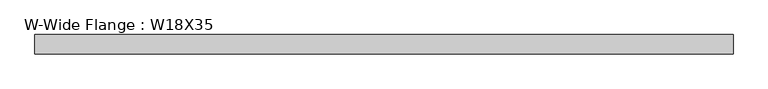
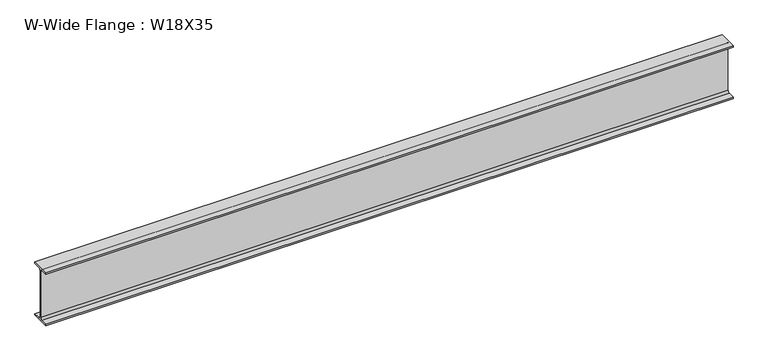
"""IFC4 building model written with IfcOpenShell, lengths in millimetres: beam geometry, W-Wide Flange : W18X35."""

from ifc_helpers import new_model, si_unit, point, frame, frame_2d, origin, place, context, project, spatial, polyline, circle_curve, trimmed, segment, composite_curve, outline, extrude, source, transform, mapped, element, save


def w_wide_flange_w18x35_70b9017d(model_context):
    return source(origin(), model_context, "Body", "SweptSolid", [
        extrude(outline(composite_curve([segment(polyline([(76.2, -213.995), (76.2, -224.79), (-76.2, -224.79), (-76.2, -213.995), (-21.59, -213.995)]), True, "CONTINUOUS"), segment(trimmed(circle_curve(frame_2d((-21.59, -196.215)), 17.78), [point((-21.59, -213.995))], [point((-3.81, -196.215))], True, "CARTESIAN"), True, "CONTINUOUS"), segment(polyline([(-3.81, -196.215), (-3.81, 196.215)]), True, "CONTINUOUS"), segment(trimmed(circle_curve(frame_2d((-21.59, 196.215)), 17.78), [point((-3.81, 196.215))], [point((-21.59, 213.995))], True, "CARTESIAN"), True, "CONTINUOUS"), segment(polyline([(-21.59, 213.995), (-76.2, 213.995), (-76.2, 224.79), (76.2, 224.79), (76.2, 213.995), (21.59, 213.995)]), True, "CONTINUOUS"), segment(trimmed(circle_curve(frame_2d((21.59, 196.215)), 17.78), [point((21.59, 213.995))], [point((3.81, 196.215))], True, "CARTESIAN"), True, "CONTINUOUS"), segment(polyline([(3.81, 196.215), (3.81, -196.215)]), True, "CONTINUOUS"), segment(trimmed(circle_curve(frame_2d((21.59, -196.215)), 17.78), [point((3.81, -196.215))], [point((21.59, -213.995))], True, "CARTESIAN"), True, "CONTINUOUS"), segment(polyline([(21.59, -213.995), (76.2, -213.995)]), True, "CONTINUOUS")], self_intersect=False)), frame((-2768.6, 0.0, 0.0), z_axis=(1.0, 0.0, 0.0), x_axis=(0.0, 1.0, 0.0)), (0.0, 0.0, 1.0), 5537.2),
    ])


if __name__ == "__main__":
    model = new_model("IFC4")
    model_context = context("Model", 3, world=origin())
    ifc_project = project(units=[si_unit("LENGTHUNIT", "METRE", prefix="MILLI")], contexts=[model_context])
    site = spatial("IfcSite", under=ifc_project)
    building = spatial("IfcBuilding", under=site)
    placement = place(None, origin())
    w_wide_flange_w18x35_shape = w_wide_flange_w18x35_70b9017d(model_context)
    element("IfcBeam", 1, ObjectType="W-Wide Flange : W18X35", at=placement, inside=building, context=model_context, shape_type="MappedRepresentation", body=[
        mapped(w_wide_flange_w18x35_shape, transform((0.0, 0.0, 0.0), x_axis=(1.0, 0.0, 0.0), y_axis=(0.0, 1.0, 0.0), z_axis=(0.0, 0.0, 1.0))),
    ])
    save(model, "model.ifc")

# Revit data of these elements
# Type "W-Wide Flange : W18X35"
#   Assembly Code = "B10"
#   W = 35
#   Length [instance default] = 5' - 0"
#   bf = 0' - 6"
#   d = 1' - 5.7"
#   k = 0' - 1 1/8"
#   k2 = 0' - 0.7"
#   tf = 0' - 0.425"
#   tw = 0' - 0.3"
#   A = 0.0715278 SF
#   Structural Material [instance default] = Steel ASTM A992
# Element 1 (IfcBeam, "W-Wide Flange : W18X35")
#   Structural Material = Steel ASTM A36
#   Materials on its faces: "Steel ASTM A36"
# Materials
#   "Steel ASTM A992": class "Metal", colour RGB 199 199 199, transparency 0, Description = "Structural steel 50ksi", Cost = 0
#   "Steel ASTM A36": class "Metal", colour RGB 199 199 199, transparency 0, Description = "Structural steel, ASTM A36 Grade B, mill finish", Cost = 0
